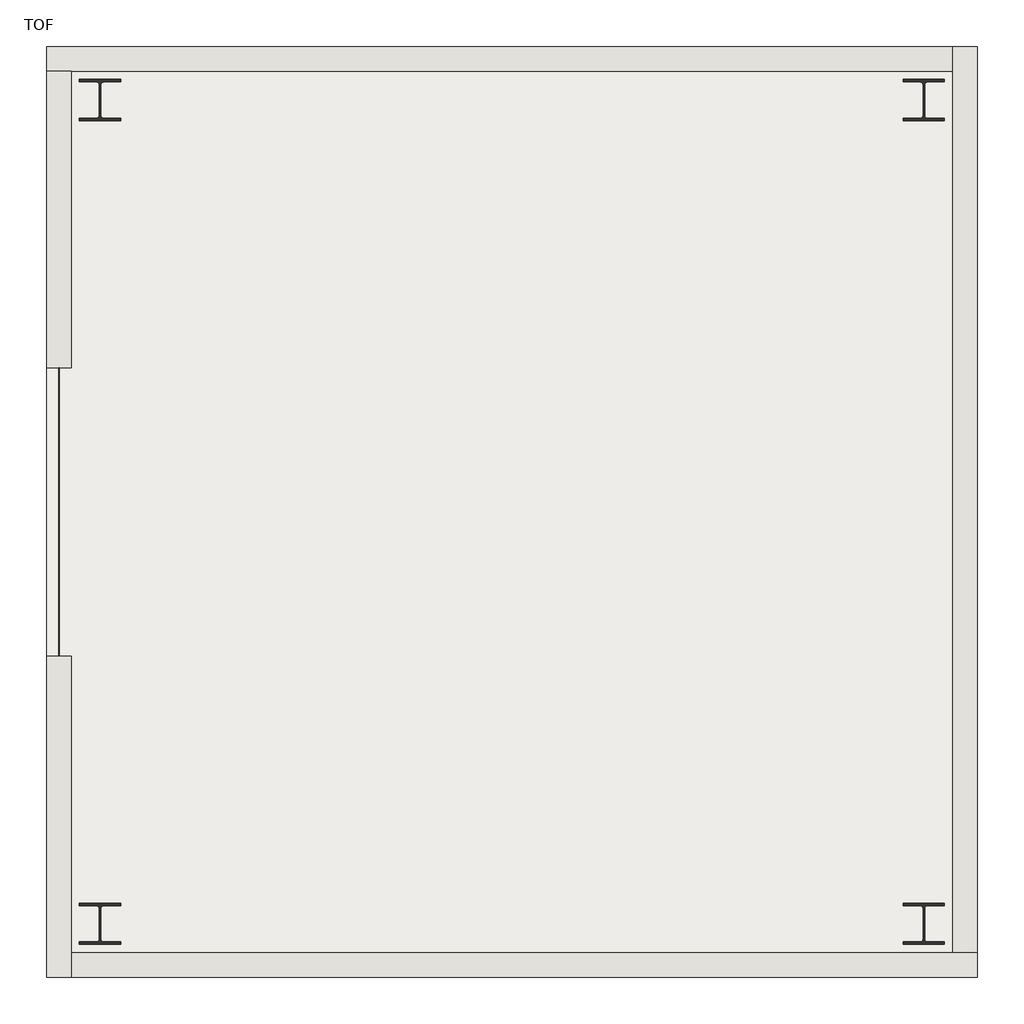
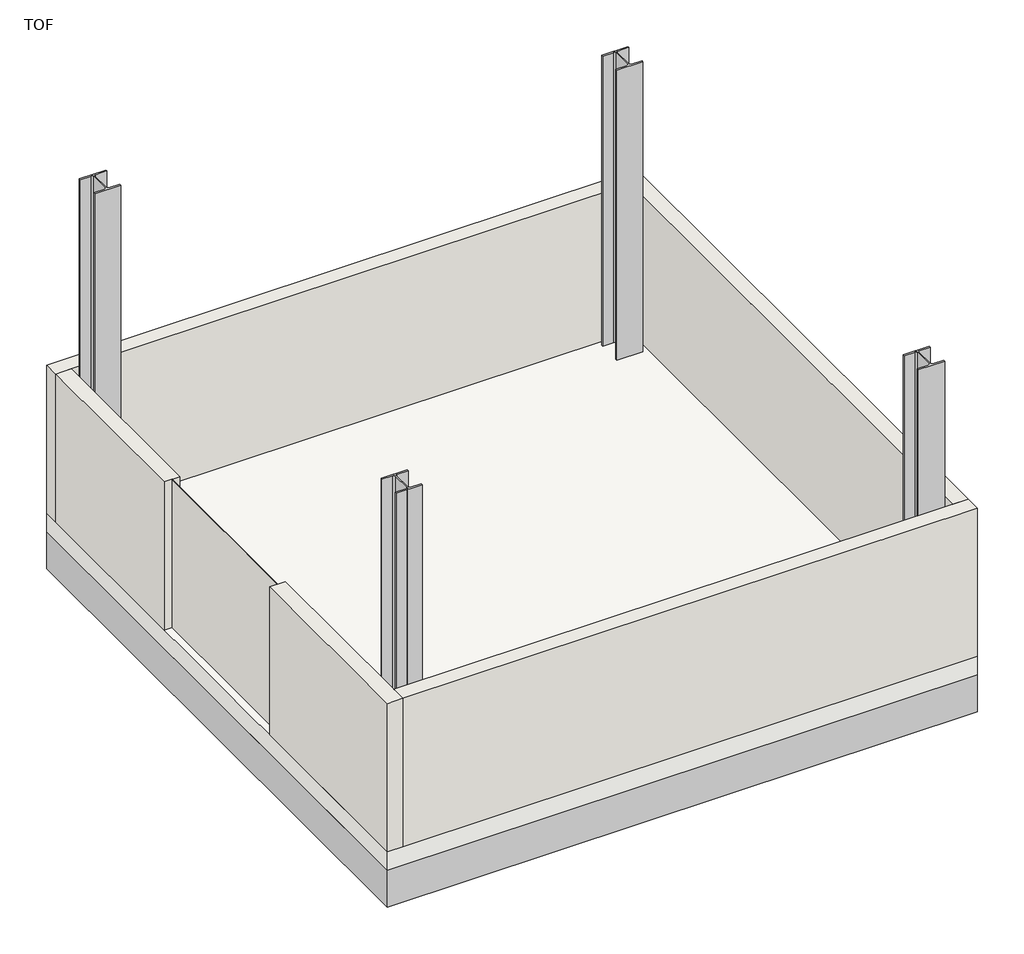
# One storey: 6 walls, 4 columns, 1 proxy, 1 slab.
"""IFC4 building model written with IfcOpenShell, lengths in millimetres."""

from ifc_helpers import new_model, si_unit, point, frame, frame_2d, origin, place, context, project, spatial, polyline, circle_curve, trimmed, segment, composite_curve, outline, extrude, faceted_brep, element, save

model = new_model("IFC4")

# Units and contexts
model_context = context("Model", 3, world=origin())
ifc_project = project(units=[si_unit("LENGTHUNIT", "METRE", prefix="MILLI")], contexts=[model_context])

# Site, building, storey
site = spatial("IfcSite", under=ifc_project)
building = spatial("IfcBuilding", under=site)
storey = spatial("IfcBuildingStorey", under=building, Name="TOF", Elevation=149.9618634)

# Proxy
placement = place(None, origin())
element("IfcBuildingElementProxy", 1, Name="H_FL_AR_S17_Thickened", ObjectType="H_FL_AR_S17_Thickened", at=placement, inside=storey, context=model_context, shape_type="Brep", body=[
    faceted_brep([(4260.0, 239.5208589, -0.0381366), (4260.0, 239.5208589, -300.0381366), (4260.0, 4759.5208589, -300.0381366), (4260.0, 4759.5208589, -0.0381366), (3660.0, 839.5208589, -0.0381366), (3660.0, 4159.5208589, -0.0381366), (3960.0, 539.5208589, -300.0381366), (3960.0, 4459.5208589, -300.0381366), (-260.0, 4759.5208589, -300.0381366), (-260.0, 4759.5208589, -0.0381366), (340.0, 4159.5208589, -0.0381366), (40.0, 4459.5208589, -300.0381366), (-260.0, 239.5208589, -300.0381366), (-260.0, 239.5208589, -0.0381366), (340.0, 839.5208589, -0.0381366), (40.0, 539.5208589, -300.0381366)], [[[0, 1, 2, 3]], [[4, 0, 3, 5]], [[6, 4, 5, 7]], [[1, 6, 7, 2]], [[3, 2, 8, 9]], [[5, 3, 9, 10]], [[7, 5, 10, 11]], [[2, 7, 11, 8]], [[9, 8, 12, 13]], [[10, 9, 13, 14]], [[11, 10, 14, 15]], [[8, 11, 15, 12]], [[13, 12, 1, 0]], [[14, 13, 0, 4]], [[15, 14, 4, 6]], [[12, 15, 6, 1]]]),
])

# Columns
element("IfcColumn", 2, ObjectType="Steel Column_H_KSD3502 : H_SC_H-200x200x8x12", at=placement, inside=storey, context=model_context, shape_type="SweptSolid", body=[
    extrude(outline(composite_curve([segment(polyline([(100.0, 599.5208589), (100.0, 587.5208589), (17.0, 587.5208589)]), True, "CONTINUOUS"), segment(trimmed(circle_curve(frame_2d((17.0, 574.5208589)), 13.0), [point((17.0, 587.5208589))], [point((4.0, 574.5208589))], True, "CARTESIAN"), True, "CONTINUOUS"), segment(polyline([(4.0, 574.5208589), (4.0, 424.5208589)]), True, "CONTINUOUS"), segment(trimmed(circle_curve(frame_2d((17.0, 424.5208589)), 13.0), [point((4.0, 424.5208589))], [point((17.0, 411.5208589))], True, "CARTESIAN"), True, "CONTINUOUS"), segment(polyline([(17.0, 411.5208589), (100.0, 411.5208589), (100.0, 399.5208589), (-100.0, 399.5208589), (-100.0, 411.5208589), (-17.0, 411.5208589)]), True, "CONTINUOUS"), segment(trimmed(circle_curve(frame_2d((-17.0, 424.5208589)), 13.0), [point((-17.0, 411.5208589))], [point((-4.0, 424.5208589))], True, "CARTESIAN"), True, "CONTINUOUS"), segment(polyline([(-4.0, 424.5208589), (-4.0, 574.5208589)]), True, "CONTINUOUS"), segment(trimmed(circle_curve(frame_2d((-17.0, 574.5208589)), 13.0), [point((-4.0, 574.5208589))], [point((-17.0, 587.5208589))], True, "CARTESIAN"), True, "CONTINUOUS"), segment(polyline([(-17.0, 587.5208589), (-100.0, 587.5208589), (-100.0, 599.5208589), (100.0, 599.5208589)]), True, "CONTINUOUS")], self_intersect=False)), frame((0.0, 0.0, 149.9618634), z_axis=(0.0, 0.0, 1.0), x_axis=(1.0, 0.0, 0.0)), (0.0, 0.0, 1.0), 2750.0),
])
element("IfcColumn", 3, ObjectType="Steel Column_H_KSD3502 : H_SC_H-200x200x8x12", at=placement, inside=storey, context=model_context, shape_type="SweptSolid", body=[
    extrude(outline(composite_curve([segment(polyline([(4100.0, 599.5208589), (4100.0, 587.5208589), (4017.0, 587.5208589)]), True, "CONTINUOUS"), segment(trimmed(circle_curve(frame_2d((4017.0, 574.5208589)), 13.0), [point((4017.0, 587.5208589))], [point((4004.0, 574.5208589))], True, "CARTESIAN"), True, "CONTINUOUS"), segment(polyline([(4004.0, 574.5208589), (4004.0, 424.5208589)]), True, "CONTINUOUS"), segment(trimmed(circle_curve(frame_2d((4017.0, 424.5208589)), 13.0), [point((4004.0, 424.5208589))], [point((4017.0, 411.5208589))], True, "CARTESIAN"), True, "CONTINUOUS"), segment(polyline([(4017.0, 411.5208589), (4100.0, 411.5208589), (4100.0, 399.5208589), (3900.0, 399.5208589), (3900.0, 411.5208589), (3983.0, 411.5208589)]), True, "CONTINUOUS"), segment(trimmed(circle_curve(frame_2d((3983.0, 424.5208589)), 13.0), [point((3983.0, 411.5208589))], [point((3996.0, 424.5208589))], True, "CARTESIAN"), True, "CONTINUOUS"), segment(polyline([(3996.0, 424.5208589), (3996.0, 574.5208589)]), True, "CONTINUOUS"), segment(trimmed(circle_curve(frame_2d((3983.0, 574.5208589)), 13.0), [point((3996.0, 574.5208589))], [point((3983.0, 587.5208589))], True, "CARTESIAN"), True, "CONTINUOUS"), segment(polyline([(3983.0, 587.5208589), (3900.0, 587.5208589), (3900.0, 599.5208589), (4100.0, 599.5208589)]), True, "CONTINUOUS")], self_intersect=False)), frame((0.0, 0.0, 149.9618634), z_axis=(0.0, 0.0, 1.0), x_axis=(1.0, 0.0, 0.0)), (0.0, 0.0, 1.0), 2350.0),
])
element("IfcColumn", 4, ObjectType="Steel Column_H_KSD3502 : H_SC_H-200x200x8x12", at=placement, inside=storey, context=model_context, shape_type="SweptSolid", body=[
    extrude(outline(composite_curve([segment(polyline([(100.0, 4599.5208589), (100.0, 4587.5208589), (17.0, 4587.5208589)]), True, "CONTINUOUS"), segment(trimmed(circle_curve(frame_2d((17.0, 4574.5208589)), 13.0), [point((17.0, 4587.5208589))], [point((4.0, 4574.5208589))], True, "CARTESIAN"), True, "CONTINUOUS"), segment(polyline([(4.0, 4574.5208589), (4.0, 4424.5208589)]), True, "CONTINUOUS"), segment(trimmed(circle_curve(frame_2d((17.0, 4424.5208589)), 13.0), [point((4.0, 4424.5208589))], [point((17.0, 4411.5208589))], True, "CARTESIAN"), True, "CONTINUOUS"), segment(polyline([(17.0, 4411.5208589), (100.0, 4411.5208589), (100.0, 4399.5208589), (-100.0, 4399.5208589), (-100.0, 4411.5208589), (-17.0, 4411.5208589)]), True, "CONTINUOUS"), segment(trimmed(circle_curve(frame_2d((-17.0, 4424.5208589)), 13.0), [point((-17.0, 4411.5208589))], [point((-4.0, 4424.5208589))], True, "CARTESIAN"), True, "CONTINUOUS"), segment(polyline([(-4.0, 4424.5208589), (-4.0, 4574.5208589)]), True, "CONTINUOUS"), segment(trimmed(circle_curve(frame_2d((-17.0, 4574.5208589)), 13.0), [point((-4.0, 4574.5208589))], [point((-17.0, 4587.5208589))], True, "CARTESIAN"), True, "CONTINUOUS"), segment(polyline([(-17.0, 4587.5208589), (-100.0, 4587.5208589), (-100.0, 4599.5208589), (100.0, 4599.5208589)]), True, "CONTINUOUS")], self_intersect=False)), frame((0.0, 0.0, 149.9618634), z_axis=(0.0, 0.0, 1.0), x_axis=(1.0, 0.0, 0.0)), (0.0, 0.0, 1.0), 2750.0),
])
element("IfcColumn", 5, ObjectType="Steel Column_H_KSD3502 : H_SC_H-200x200x8x12", at=placement, inside=storey, context=model_context, shape_type="SweptSolid", body=[
    extrude(outline(composite_curve([segment(polyline([(4100.0, 4599.5208589), (4100.0, 4587.5208589), (4017.0, 4587.5208589)]), True, "CONTINUOUS"), segment(trimmed(circle_curve(frame_2d((4017.0, 4574.5208589)), 13.0), [point((4017.0, 4587.5208589))], [point((4004.0, 4574.5208589))], True, "CARTESIAN"), True, "CONTINUOUS"), segment(polyline([(4004.0, 4574.5208589), (4004.0, 4424.5208589)]), True, "CONTINUOUS"), segment(trimmed(circle_curve(frame_2d((4017.0, 4424.5208589)), 13.0), [point((4004.0, 4424.5208589))], [point((4017.0, 4411.5208589))], True, "CARTESIAN"), True, "CONTINUOUS"), segment(polyline([(4017.0, 4411.5208589), (4100.0, 4411.5208589), (4100.0, 4399.5208589), (3900.0, 4399.5208589), (3900.0, 4411.5208589), (3983.0, 4411.5208589)]), True, "CONTINUOUS"), segment(trimmed(circle_curve(frame_2d((3983.0, 4424.5208589)), 13.0), [point((3983.0, 4411.5208589))], [point((3996.0, 4424.5208589))], True, "CARTESIAN"), True, "CONTINUOUS"), segment(polyline([(3996.0, 4424.5208589), (3996.0, 4574.5208589)]), True, "CONTINUOUS"), segment(trimmed(circle_curve(frame_2d((3983.0, 4574.5208589)), 13.0), [point((3996.0, 4574.5208589))], [point((3983.0, 4587.5208589))], True, "CARTESIAN"), True, "CONTINUOUS"), segment(polyline([(3983.0, 4587.5208589), (3900.0, 4587.5208589), (3900.0, 4599.5208589), (4100.0, 4599.5208589)]), True, "CONTINUOUS")], self_intersect=False)), frame((0.0, 0.0, 149.9618634), z_axis=(0.0, 0.0, 1.0), x_axis=(1.0, 0.0, 0.0)), (0.0, 0.0, 1.0), 2350.0),
])

# Slab
element("IfcSlab", 6, ObjectType="H_FL_AR_S17_RC Slab T150", at=placement, inside=storey, context=model_context, shape_type="SweptSolid", body=[
    extrude(outline(polyline([(4260.0, 239.5208589), (-260.0, 239.5208589), (-260.0, 4759.5208589), (4260.0, 4759.5208589), (4260.0, 239.5208589)])), frame((0.0, 0.0, -0.0381366), z_axis=(0.0, 0.0, 1.0), x_axis=(1.0, 0.0, 0.0)), (0.0, 0.0, 1.0), 150.0),
])

# Walls
element("IfcWall", 7, ObjectType="H_WA_AR_B02_Ext Wall_1L Gypsum_1B Brick_Glass Wool", at=placement, inside=storey, context=model_context, shape_type="Brep", body=[
    faceted_brep([(-260.0, 4639.5208589, 149.9618634), (-140.0, 4639.5208589, 149.9618634), (4140.0, 4639.5208589, 149.9618634), (4140.0, 4639.5208589, 1349.9618634), (-140.0, 4639.5208589, 1349.9618634), (-260.0, 4639.5208589, 1349.9618634), (-260.0, 4759.5208589, 149.9618634), (-260.0, 4759.5208589, 1349.9618634), (4140.0, 4759.5208589, 1349.9618634), (4140.0, 4759.5208589, 149.9618634)], [[[0, 1, 2, 3, 4, 5]], [[6, 7, 8, 9]], [[2, 1, 0, 6, 9]], [[5, 4, 3, 8, 7]], [[0, 5, 7, 6]], [[3, 2, 9, 8]]]),
])
element("IfcWall", 8, ObjectType="H_WA_AR_B02_Ext Wall_1L Gypsum_1B Brick_Glass Wool", at=placement, inside=storey, context=model_context, shape_type="Brep", body=[
    faceted_brep([(-140.0, 239.5208589, 149.9618634), (-140.0, 359.5208589, 149.9618634), (-140.0, 1799.5208589, 149.9618634), (-140.0, 1799.5208589, 1349.9618634), (-140.0, 359.5208589, 1349.9618634), (-140.0, 239.5208589, 1349.9618634), (-260.0, 239.5208589, 149.9618634), (-260.0, 239.5208589, 1349.9618634), (-260.0, 1799.5208589, 1349.9618634), (-260.0, 1799.5208589, 149.9618634)], [[[0, 1, 2, 3, 4, 5]], [[6, 7, 8, 9]], [[2, 1, 0, 6, 9]], [[3, 2, 9, 8]], [[5, 4, 3, 8, 7]], [[0, 5, 7, 6]]]),
])
element("IfcWall", 9, ObjectType="H_WA_AR_B02_Ext Wall_1L Gypsum_1B Brick_Glass Wool", at=placement, inside=storey, context=model_context, shape_type="Brep", body=[
    faceted_brep([(4260.0, 359.5208589, 149.9618634), (4140.0, 359.5208589, 149.9618634), (-140.0, 359.5208589, 149.9618634), (-140.0, 359.5208589, 1349.9618634), (4140.0, 359.5208589, 1349.9618634), (4260.0, 359.5208589, 1349.9618634), (4260.0, 239.5208589, 149.9618634), (4260.0, 239.5208589, 1349.9618634), (-140.0, 239.5208589, 1349.9618634), (-140.0, 239.5208589, 149.9618634)], [[[0, 1, 2, 3, 4, 5]], [[6, 7, 8, 9]], [[2, 1, 0, 6, 9]], [[5, 4, 3, 8, 7]], [[0, 5, 7, 6]], [[3, 2, 9, 8]]]),
])
element("IfcWall", 10, ObjectType="H_WA_AR_B02_Ext Wall_1L Gypsum_1B Brick_Glass Wool", at=placement, inside=storey, context=model_context, shape_type="Brep", body=[
    faceted_brep([(4140.0, 4759.5208589, 149.9618634), (4140.0, 4639.5208589, 149.9618634), (4140.0, 359.5208589, 149.9618634), (4140.0, 359.5208589, 1349.9618634), (4140.0, 4639.5208589, 1349.9618634), (4140.0, 4759.5208589, 1349.9618634), (4260.0, 4759.5208589, 149.9618634), (4260.0, 4759.5208589, 1349.9618634), (4260.0, 359.5208589, 1349.9618634), (4260.0, 359.5208589, 149.9618634)], [[[0, 1, 2, 3, 4, 5]], [[6, 7, 8, 9]], [[2, 1, 0, 6, 9]], [[5, 4, 3, 8, 7]], [[0, 5, 7, 6]], [[3, 2, 9, 8]]]),
])
element("IfcWall", 11, ObjectType="H_WA_AR_B02_Ext Wall_1L Gypsum_1B Brick_Glass Wool", at=placement, inside=storey, context=model_context, shape_type="SweptSolid", body=[
    extrude(outline(polyline([(-140.0, 4639.5208589), (-140.0, 3199.5208589), (-260.0, 3199.5208589), (-260.0, 4639.5208589), (-140.0, 4639.5208589)])), frame((0.0, 0.0, 149.9618634), z_axis=(0.0, 0.0, 1.0), x_axis=(1.0, 0.0, 0.0)), (0.0, 0.0, 1.0), 1200.0),
])
element("IfcWall", 12, ObjectType="H_WA_AR_B02_Wall Single Sheet_T0.7", at=placement, inside=storey, context=model_context, shape_type="SweptSolid", body=[
    extrude(outline(polyline([(-200.5, 1799.5208589), (-200.5, 3199.5208589), (-199.5, 3199.5208589), (-199.5, 1799.5208589), (-200.5, 1799.5208589)])), frame((0.0, 0.0, 149.9618634), z_axis=(0.0, 0.0, 1.0), x_axis=(1.0, 0.0, 0.0)), (0.0, 0.0, 1.0), 1200.0),
])

save(model, "model.ifc")

# Revit data of these elements
# Project information
#   H_Seismic Condition = "A as per ASCE 7-10"
#   H_Soil Condition = "C as per ASCE 7-10"
#   H_Basic Wind Speed = "58.3m/s ASCE7-10"
#   H_DS Project Code = "FAASA2302"
#   H_Project Abbreviation = "SACE2"
#   H_Project Division = "화공"
#   H_Project Finish = "2027-03-05"
#   H_Project Location = "Jafurah, Saudi Arabia"
#   H_Project Start = "2024-01-03"
#   H_Project Type = "EPC"
#   H_Smart Code = "FAASA2302"
#   Project Issue Date = "Issue Date"
#   Project Status = "Project Status"
#   Client Name = "Owner"
#   Project Address = "Enter address here"
#   Project Name = "Project Name"
#   Project Number = "0001"
# Grids (mm)
#   "Y2": line (-3860.098, 499.521) -> (12335.324, 499.521)
#   "X1": line (0, 9877.337) -> (0, -6208.346)
#   "X2": line (4000, 9877.337) -> (4000, -6208.346)
#   "Y1": line (-3860.098, 4499.521) -> (12335.324, 4499.521)
# Type "Steel Column_H_KSD3502 : H_SC_H-200x200x8x12"
#   Width = 20.0 cm
#   Web Thickness = 0.8 cm
#   Web Fillet = 1.3 cm
#   Warping Constant = 141376.0 cm⁶
#   Torsional Moment of Inertia = 26.2485 cm⁴
#   Section Area = 63.53 cm²
#   Plastic Modulus weak axis = 244.0 cm³
#   Plastic Modulus strong axis = 525.0 cm³
#   Perimeter = 1.16 m²/m
#   Nominal Weight = 49.90 kgf/m
#   Moment of Inertia weak axis = 1600.00 cm⁴
#   Moment of Inertia strong axis = 4720.00 cm⁴
#   Height = 20.0 cm
#   Flange Thickness = 1.2 cm
#   Elastic Modulus weak axis = 160.0 cm³
#   Elastic Modulus strong axis = 472.0 cm³
#   Centroid Vertical = 10.0 cm
#   Centroid Horizontal = 10.0 cm
#   Structural Material [instance default] = Steel, 45-345
#   Section Name Key = ""
#   Bolt Spacing = 0
#   Assembly Code = ""
# Type "H_FL_AR_S17_RC Slab T150"
#   Keynote = ""
#   Type Comments = ""
#   Description = ""
#   Function = 1
#   Layers, outside or top first: 150 mm no material (function 1)
# Type "H_WA_AR_B02_Ext Wall_1L Gypsum_1B Brick_Glass Wool"
#   Type Comments = "구조_콘크리트"
#   Layers, outside or top first: 120 mm no material (function 1)
# Type "H_WA_AR_B02_Wall Single Sheet_T0.7"
#   Type Comments = "구조_콘크리트"
#   Layers, outside or top first: 0 mm no material (function 100); 1 mm no material (function 4); 0 mm no material (function 100)
# Element 1 (IfcBuildingElementProxy, "H_FL_AR_S17_Thickened")
#   Phase Created = New Construction
#   Materials on its faces: "Default Floor"
# Elements 2, 3, 4, 5 (IfcColumn, "Steel Column_H_KSD3502 : H_SC_H-200x200x8x12")
#   Comments = ""
#   Structural Material = none
#   Phase Created = New Construction
# Element 6 (IfcSlab, "H_FL_AR_S17_RC Slab T150")
#   Height Offset From Level = 0 mm
#   Phase Created = New Construction
#   Materials on its faces: "Default Floor"
# Elements 7, 8, 9, 10, 11 (IfcWall, "H_WA_AR_B02_Ext Wall_1L Gypsum_1B Brick_Glass Wool")
#   Top Offset = 0 mm
#   Base Offset = 0 mm
#   Unconnected Height = 1200 mm
#   wall height = 1200 mm
#   Phase Created = New Construction
#   Base Constraint = TOF
#   Materials on its faces: "Default Wall"
# Element 12 (IfcWall, "H_WA_AR_B02_Wall Single Sheet_T0.7")
#   Top Offset = 0 mm
#   Base Offset = 0 mm
#   Unconnected Height = 1200 mm
#   wall height = 1200 mm
#   Phase Created = New Construction
#   Base Constraint = TOF
#   Materials on its faces: "Default Wall"
# Materials
#   "Steel, 45-345": class "Metal", colour RGB 189 187 185, transparency 0, Description = "Steel 345 MPa", Cost = 0
#   "Default Floor": class "Miscellaneous", colour RGB 80 80 80, transparency 0
#   "Default Wall": class "Miscellaneous", colour RGB 80 80 80, transparency 0
# Room at (2078.173, 2915.248) mm, phase "New Construction", upper level "TOC", upper offset 1000 mm, lower offset -1000 mm
#   Comments = ""
#   Number = "126"
#   Name = "SHELTER AREA"
